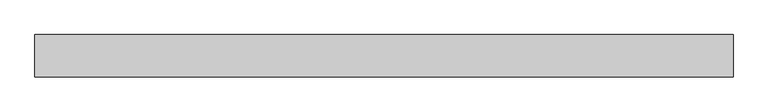
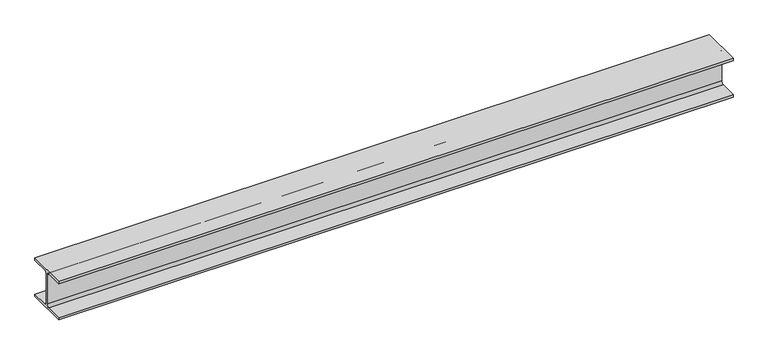
"""IFC4 building model written with IfcOpenShell, lengths in millimetres: beam geometry, 0912_Steel Framing_H-KSD3502 : H_SB_ASB_H-200x200x8x12."""

from ifc_helpers import new_model, si_unit, point, frame, frame_2d, origin, place, context, project, spatial, polyline, circle_curve, trimmed, segment, composite_curve, outline, extrude, source, transform, mapped, element, save


def beam_d7d6f078(model_context):
    return source(origin(), model_context, "Body", "SweptSolid", [
        extrude(outline(composite_curve([segment(polyline([(100.0, -88.0), (100.0, -100.0), (-100.0, -100.0), (-100.0, -88.0), (-17.0, -88.0)]), True, "CONTINUOUS"), segment(trimmed(circle_curve(frame_2d((-17.0, -75.0)), 13.0), [point((-17.0, -88.0))], [point((-4.0, -75.0))], True, "CARTESIAN"), True, "CONTINUOUS"), segment(polyline([(-4.0, -75.0), (-4.0, 75.0)]), True, "CONTINUOUS"), segment(trimmed(circle_curve(frame_2d((-17.0, 75.0)), 13.0), [point((-4.0, 75.0))], [point((-17.0, 88.0))], True, "CARTESIAN"), True, "CONTINUOUS"), segment(polyline([(-17.0, 88.0), (-100.0, 88.0), (-100.0, 100.0), (100.0, 100.0), (100.0, 88.0), (17.0, 88.0)]), True, "CONTINUOUS"), segment(trimmed(circle_curve(frame_2d((17.0, 75.0)), 13.0), [point((17.0, 88.0))], [point((4.0, 75.0))], True, "CARTESIAN"), True, "CONTINUOUS"), segment(polyline([(4.0, 75.0), (4.0, -75.0)]), True, "CONTINUOUS"), segment(trimmed(circle_curve(frame_2d((17.0, -75.0)), 13.0), [point((4.0, -75.0))], [point((17.0, -88.0))], True, "CARTESIAN"), True, "CONTINUOUS"), segment(polyline([(17.0, -88.0), (100.0, -88.0)]), True, "CONTINUOUS")], self_intersect=False)), frame((-1704.6789218, 0.0, 0.0), z_axis=(1.0, 0.0, 0.0), x_axis=(0.0, 1.0, 0.0)), (0.0, 0.0, 1.0), 3300.6879746),
    ])


if __name__ == "__main__":
    model = new_model("IFC4")
    model_context = context("Model", 3, world=origin())
    ifc_project = project(units=[si_unit("LENGTHUNIT", "METRE", prefix="MILLI")], contexts=[model_context])
    site = spatial("IfcSite", under=ifc_project)
    building = spatial("IfcBuilding", under=site)
    placement = place(None, origin())
    beam_shape = beam_d7d6f078(model_context)
    element("IfcBeam", 1, ObjectType="0912_Steel Framing_H-KSD3502 : H_SB_ASB_H-200x200x8x12", at=placement, inside=building, context=model_context, shape_type="MappedRepresentation", body=[
        mapped(beam_shape, transform((0.0, 0.0, 0.0), x_axis=(1.0, 0.0, 0.0), y_axis=(0.0, 1.0, 0.0), z_axis=(0.0, 0.0, 1.0))),
    ])
    save(model, "model.ifc")

# Revit data of these elements
# Type "0912_Steel Framing_H-KSD3502 : H_SB_ASB_H-200x200x8x12"
#   H_WM Code_1 = "S01AA002-00001 | Main Steel Structure Fabrication Work | Shelter/Building | Medium Steel - Standard (90KG/M>Weight≥30KG/M) | Material: (   )"
#   H_WM Code_2 = "S03AA028-00001 | Main Steel Structure Erection Work | Shelter/Building | Medium Steel (90KG/M>Weight≥30KG/M) | Material: (   )"
#   H_WM Code_3 = "S01AA010-00001 | Main Steel Structure Fabrication Work | Shelter/Building | Steel Painting/Coating | for Non-Fireproofed Steel Surface, Surface Preparation, Primer, Second & Final Coat | Material: (   )"
#   H_Q'ty Cal Type Tag = "SB-Q2"
#   Width = 20.0 cm
#   Web Thickness = 0.8 cm
#   Web Fillet = 1.3 cm
#   Warping Constant = 141000.0 cm⁶
#   W = 0
#   Torsional Moment of Inertia = 26.2485 cm⁴
#   Section Area = 63.53 cm²
#   Plastic Modulus weak axis = 244.0 cm³
#   Plastic Modulus strong axis = 525.0 cm³
#   Perimeter = 1.16 m²/m
#   Nominal Weight = 49.90 kgf/m
#   Moment of Inertia weak axis = 1600.00 cm⁴
#   Moment of Inertia strong axis = 4720.00 cm⁴
#   Height = 20.0 cm
#   Flange Thickness = 1.2 cm
#   Elastic Modulus weak axis = 160.0 cm³
#   Elastic Modulus strong axis = 472.0 cm³
#   Centroid Vertical = 10.0 cm
#   Centroid Horizontal = 10.0 cm
#   Ix = 47200000
#   Length [instance default] = 1.5240 m
#   Zx = 525000
#   b = 0.2000 m
#   h = 0.2000 m
#   r = 0.0130 m
#   s = 0.0080 m
#   t = 0.0120 m
#   A = 0.006353 m²
#   Structural Material [instance default] = Steel, 45-345
#   Assembly Code = ""
# Element 1 (IfcBeam, "0912_Steel Framing_H-KSD3502 : H_SB_ASB_H-200x200x8x12")
#   Structural Material = none
# Materials
#   "Steel, 45-345": class "Metal", colour RGB 189 187 185, transparency 0, Description = "Steel 345 MPa", Cost = 0
